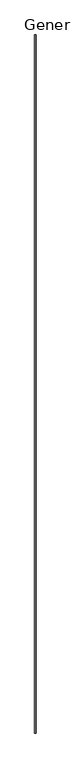
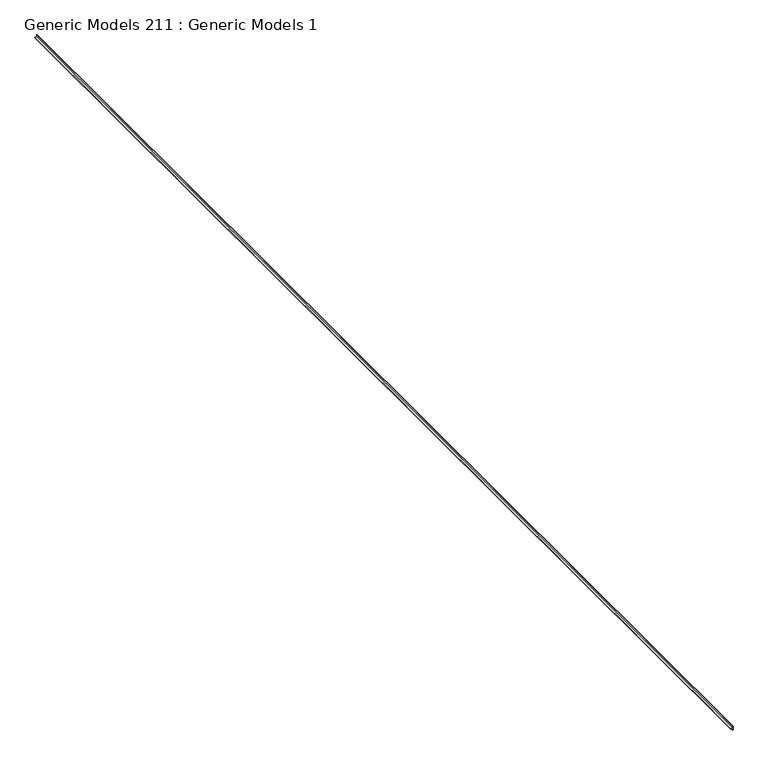
"""IFC4 building model written with IfcOpenShell, lengths in millimetres: proxy geometry, Generic Models 211 : Generic Models 1."""

from ifc_helpers import new_model, si_unit, origin, place, context, project, spatial, faceted_brep, source, transform, mapped, element, save


def generic_models_211_generic_models_1_211f5ff2(model_context):
    return source(origin(), model_context, "Body", "Brep", [
        faceted_brep([(-6625.8562339, 11981.8769662, 126342.521), (-6625.8562339, 11981.8769662, 126303.151), (-6627.1262339, 11981.8769662, 126303.151), (-6627.1262339, 11981.8769662, 126322.201), (-6646.8112339, 11981.8769662, 126322.201), (-6646.8112339, 11981.8769662, 126318.7212), (-6648.0812339, 11981.8769662, 126318.7212), (-6648.0812339, 11981.8769662, 126323.471), (-6627.1262339, 11981.8769662, 126323.471), (-6627.1262339, 11981.8769662, 126342.521), (-6625.8562339, -464.1230338, 126342.521), (-6627.1262339, -464.1230338, 126342.521), (-6627.1262339, -464.1230338, 126323.471), (-6648.0812339, -464.1230338, 126323.471), (-6648.0812339, -464.1230338, 126318.7212), (-6646.8112339, -464.1230338, 126318.7212), (-6646.8112339, -464.1230338, 126322.201), (-6629.7612592, -464.1230338, 126322.201), (-6627.1262339, -464.1230338, 126322.201), (-6627.1262339, -464.1230338, 126303.151), (-6625.8562339, -464.1230338, 126303.151), (-6648.0812339, 11778.6769662, 126318.7212), (-6646.8112339, 11778.6769662, 126318.7212), (-6646.8112339, 11778.6769662, 126322.201)], [[[0, 1, 2, 3, 4, 5, 6, 7, 8, 9]], [[10, 11, 12, 13, 14, 15, 16, 17, 18, 19, 20]], [[0, 9, 11, 10]], [[9, 8, 12, 11]], [[8, 7, 13, 12]], [[7, 6, 21, 14, 13]], [[6, 5, 22, 15, 14, 21]], [[5, 4, 23, 16, 15, 22]], [[4, 3, 18, 17, 16, 23]], [[3, 2, 19, 18]], [[2, 1, 20, 19]], [[1, 0, 10, 20]]]),
    ])


if __name__ == "__main__":
    model = new_model("IFC4")
    model_context = context("Model", 3, world=origin())
    ifc_project = project(units=[si_unit("LENGTHUNIT", "METRE", prefix="MILLI")], contexts=[model_context])
    site = spatial("IfcSite", under=ifc_project)
    building = spatial("IfcBuilding", under=site)
    placement = place(None, origin())
    generic_models_211_generic_models_1_shape = generic_models_211_generic_models_1_211f5ff2(model_context)
    element("IfcBuildingElementProxy", 1, Name="Generic Models 211 : Generic Models 1", ObjectType="Generic Models 211 : Generic Models 1", at=placement, inside=building, context=model_context, shape_type="MappedRepresentation", body=[
        mapped(generic_models_211_generic_models_1_shape, transform((0.0, 0.0, 0.0), x_axis=(1.0, 0.0, 0.0), y_axis=(0.0, 1.0, 0.0), z_axis=(0.0, 0.0, 1.0))),
    ])
    save(model, "model.ifc")

# Revit data of these elements
# Element 1 (IfcBuildingElementProxy, "Generic Models 211 : Generic Models 1")
#   Materials on its faces: "_ 16 GA. COPPER VENTED T REVEAL BEAD (CONT. AROUND PERIMETER OF BEAM)"
# Materials
#   "_ 16 GA. COPPER VENTED T REVEAL BEAD (CONT. AROUND PERIMETER OF BEAM)": class "Generic", colour RGB 253 192 103, transparency 0, Cost = 0
